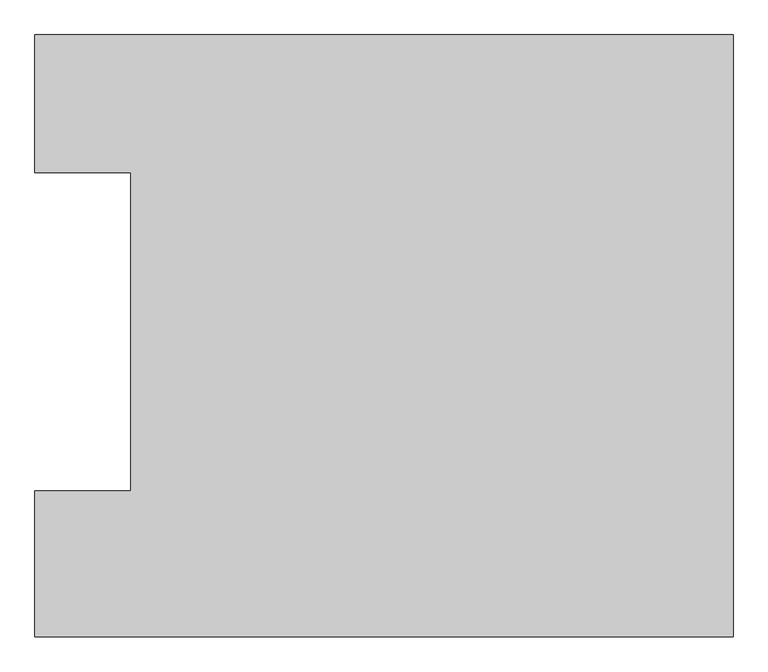
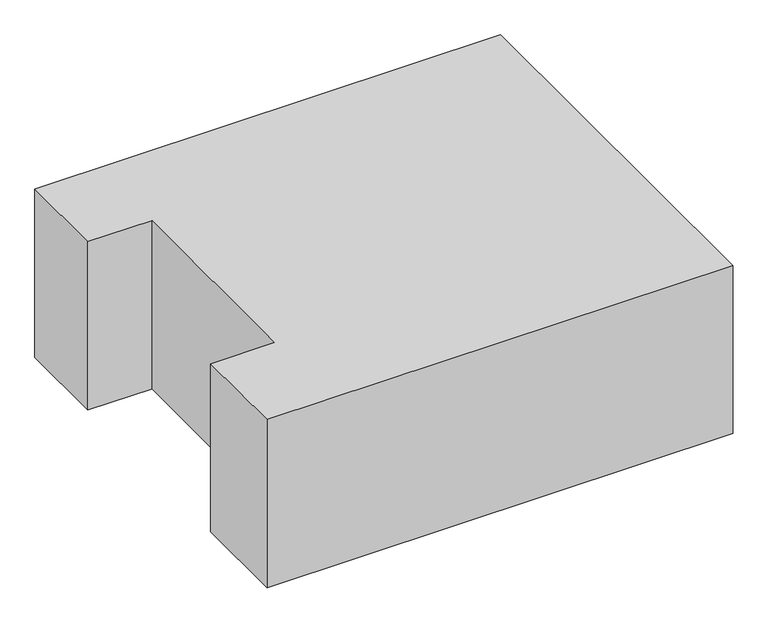
"""IFC4 building model written with IfcOpenShell, lengths in millimetres: proxy geometry, 0_3d."""

import ifcopenshell
import ifcopenshell.guid

model = None  # the IFC model being written
_history = None  # IfcOwnerHistory: only IFC2X3 demands one
_inside = {}  # id of a spatial element -> (the spatial element, [elements in it])
_under = {}  # id of a project, library or spatial element -> (it, [spatial elements below it])
_declared = {}  # id of a project -> (the project, [libraries it declares])
_typed = {}  # id of a type object -> (the type object, [elements of that type])
_made_of = {}  # id of a material, layer set ... -> (it, [elements and type objects made of it])


def new_model(schema):
    """Start an empty IFC model of exactly this schema.

    Asked for "IFC4X3", IfcOpenShell would pick the latest addendum, in which some entities
    have other attributes; the version numbers below select the first issue.
    IFC2X3 requires an IfcOwnerHistory on every rooted entity: one is made here for all.
    """
    global model, _history
    if schema == "IFC4X3":
        model = ifcopenshell.file(schema_version=(4, 3, 0, 0))
    else:
        model = ifcopenshell.file(schema=schema)
    _inside.clear()
    _under.clear()
    _declared.clear()
    _typed.clear()
    _made_of.clear()
    _history = None
    if model.schema == "IFC2X3":
        org = make("IfcOrganization", Name="unknown")
        user = make(
            "IfcPersonAndOrganization",
            ThePerson=make("IfcPerson", FamilyName="unknown"),
            TheOrganization=org,
        )
        app = make(
            "IfcApplication",
            ApplicationDeveloper=org,
            Version="unknown",
            ApplicationFullName="unknown",
            ApplicationIdentifier="unknown",
        )
        _history = make(
            "IfcOwnerHistory",
            OwningUser=user,
            OwningApplication=app,
            ChangeAction="ADDED",
            CreationDate=0,
        )
    return model


def make(cls, **values):
    """One entity of the class cls with the attributes given. An attribute that is None is left unset."""
    return model.create_entity(
        cls, **{name: value for name, value in values.items() if value is not None}
    )


def rooted(cls, **values):
    """An entity with a GlobalId (a new one), such as an element, a storey or a relation."""
    return make(cls, GlobalId=ifcopenshell.guid.new(), OwnerHistory=_history, **values)


def si_unit(unit_type, name, prefix=None):
    """IfcSIUnit, for example si_unit("LENGTHUNIT", "METRE", prefix="MILLI")."""
    return make("IfcSIUnit", UnitType=unit_type, Prefix=prefix, Name=name)


def assignment(units):
    """IfcUnitAssignment: the units of a project."""
    return None if units is None else make("IfcUnitAssignment", Units=units)


def point(xyz):
    """IfcCartesianPoint."""
    return None if xyz is None else make("IfcCartesianPoint", Coordinates=xyz)


def direction(xyz):
    """IfcDirection."""
    return None if xyz is None else make("IfcDirection", DirectionRatios=xyz)


def frame(location, z_axis=None, x_axis=None):
    """IfcAxis2Placement3D, a coordinate frame: its origin and axes. An axis left out is left unset."""
    return make(
        "IfcAxis2Placement3D",
        Location=point(location),
        Axis=direction(z_axis),
        RefDirection=direction(x_axis),
    )


def origin():
    """The frame at (0, 0, 0) with its axes left unset."""
    return frame((0.0, 0.0, 0.0))


def origin_with_axes():
    """The frame at (0, 0, 0) with the z axis (0, 0, 1) and the x axis (1, 0, 0) written out."""
    return frame((0.0, 0.0, 0.0), z_axis=(0.0, 0.0, 1.0), x_axis=(1.0, 0.0, 0.0))


def place(relative_to, where):
    """IfcLocalPlacement: puts the frame where relative to a parent placement (None: the world)."""
    return make(
        "IfcLocalPlacement", PlacementRelTo=relative_to, RelativePlacement=where
    )


def context(
    kind, dimensions, precision=None, world=None, true_north=None, identifier=None
):
    """IfcGeometricRepresentationContext, for example the 3D "Model" context."""
    return make(
        "IfcGeometricRepresentationContext",
        ContextIdentifier=identifier,
        ContextType=kind,
        CoordinateSpaceDimension=dimensions,
        Precision=precision,
        WorldCoordinateSystem=world,
        TrueNorth=true_north,
    )


def project(units=None, contexts=None):
    """IfcProject with its units and contexts."""
    return rooted(
        "IfcProject",
        Name="project",
        RepresentationContexts=contexts,
        UnitsInContext=assignment(units),
    )


def spatial(cls, under=None, at=None, **own):
    """A site, building, storey or space (cls), placed at a placement, below another one or the project."""
    s = rooted(cls, ObjectPlacement=at, **own)
    if under is not None:
        _under.setdefault(under.id(), (under, []))[1].append(s)
    return s


def polyline(points):
    """IfcPolyline through the points."""
    return make("IfcPolyline", Points=[point(p) for p in points])


def outline(outer, holes=None, kind="AREA"):
    """IfcArbitraryClosedProfileDef: a profile drawn as a closed curve; with holes, ...WithVoids."""
    if holes is None:
        return make("IfcArbitraryClosedProfileDef", ProfileType=kind, OuterCurve=outer)
    return make(
        "IfcArbitraryProfileDefWithVoids",
        ProfileType=kind,
        OuterCurve=outer,
        InnerCurves=holes,
    )


def extrude(swept, where, along, depth):
    """IfcExtrudedAreaSolid: the profile swept, set in the frame where, extruded along a direction by depth."""
    return make(
        "IfcExtrudedAreaSolid",
        SweptArea=swept,
        Position=where,
        ExtrudedDirection=direction(along),
        Depth=depth,
    )


def shape(context_of_items, identifier, shape_type, items):
    """IfcShapeRepresentation: the items that make up one representation, for example the "Body"."""
    return make(
        "IfcShapeRepresentation",
        ContextOfItems=context_of_items,
        RepresentationIdentifier=identifier,
        RepresentationType=shape_type,
        Items=items,
    )


def source(mapping_origin, context_of_items, identifier, shape_type, items):
    """IfcRepresentationMap: a shape defined once, which mapped items show again and again."""
    return make(
        "IfcRepresentationMap",
        MappingOrigin=mapping_origin,
        MappedRepresentation=shape(context_of_items, identifier, shape_type, items),
    )


def transform(
    local_origin,
    x_axis=None,
    y_axis=None,
    z_axis=None,
    scale=None,
    scale2=None,
    scale3=None,
    uniform=True,
):
    """IfcCartesianTransformationOperator3D, or its non-uniform kind. x_axis, y_axis, z_axis: its Axis1, 2, 3."""
    if uniform:
        return make(
            "IfcCartesianTransformationOperator3D",
            Axis1=direction(x_axis),
            Axis2=direction(y_axis),
            LocalOrigin=point(local_origin),
            Scale=scale,
            Axis3=direction(z_axis),
        )
    return make(
        "IfcCartesianTransformationOperator3DnonUniform",
        Axis1=direction(x_axis),
        Axis2=direction(y_axis),
        LocalOrigin=point(local_origin),
        Scale=scale,
        Axis3=direction(z_axis),
        Scale2=scale2,
        Scale3=scale3,
    )


def mapped(mapping_source, mapping_target):
    """IfcMappedItem: shows the shape of a source again, moved by a transform."""
    return make(
        "IfcMappedItem", MappingSource=mapping_source, MappingTarget=mapping_target
    )


def made_of(thing, what):
    """Note that an element or type object is made of a material, layer set ...; save() writes the relation."""
    if what is not None:
        _made_of.setdefault(what.id(), (what, []))[1].append(thing)
    return thing


def element(
    cls,
    number,
    at=None,
    inside=None,
    cuts=None,
    type_object=None,
    material=None,
    context=None,
    identifier="Body",
    shape_type=None,
    held_by="IfcProductDefinitionShape",
    body=None,
    shapes=None,
    **own,
):
    """One element of the class cls, such as IfcWall. Its Tag is "e" and its number.

    at: its placement. inside: the storey or other place that contains it. cuts: it is an
    opening in that element (IfcRelVoidsElement). A single representation is given by context,
    identifier, shape_type and body (its items); several are given by shapes. held_by: the class
    of the entity that holds the representations. save() writes the other relations.
    """
    e = rooted(cls, Tag="e%d" % number, ObjectPlacement=at, **own)
    if body is not None:
        shapes = [shape(context, identifier, shape_type, body)]
    if shapes is not None:
        e.Representation = make(held_by, Representations=shapes)
    if inside is not None:
        _inside.setdefault(inside.id(), (inside, []))[1].append(e)
    if cuts is not None:
        rooted(
            "IfcRelVoidsElement", RelatingBuildingElement=cuts, RelatedOpeningElement=e
        )
    if type_object is not None:
        _typed.setdefault(type_object.id(), (type_object, []))[1].append(e)
    return made_of(e, material)


def aggregate(whole, parts):
    """IfcRelAggregates: a whole, such as a stair, and the parts it consists of."""
    return rooted("IfcRelAggregates", RelatingObject=whole, RelatedObjects=parts)


def save(model, path):
    """Write the relations noted so far, then the file.

    IfcRelAggregates (storeys below a building ...), IfcRelContainedInSpatialStructure (elements
    in a storey), IfcRelDefinesByType, IfcRelAssociatesMaterial and IfcRelDeclares: one each for
    every whole, place, type object, material and project.
    """
    for whole, parts in _under.values():
        aggregate(whole, parts)
    for where, things in _inside.values():
        rooted(
            "IfcRelContainedInSpatialStructure",
            RelatedElements=things,
            RelatingStructure=where,
        )
    for kind, things in _typed.values():
        rooted("IfcRelDefinesByType", RelatedObjects=things, RelatingType=kind)
    for what, things in _made_of.values():
        rooted("IfcRelAssociatesMaterial", RelatedObjects=things, RelatingMaterial=what)
    for by, libraries in _declared.values():
        rooted("IfcRelDeclares", RelatingContext=by, RelatedDefinitions=libraries)
    model.write(path)


def generic_models_1e1fada3(model_context):
    return source(origin(), model_context, "Body", "SweptSolid", [
        extrude(outline(polyline([(0.0, 0.0), (0.0, 1367.8), (900.0, 1367.8), (900.0, 4357.8), (0.0, 4357.8), (0.0, 5650.0), (6550.0, 5650.0), (6550.0, 0.0), (0.0, 0.0)])), origin_with_axes(), (0.0, 0.0, 1.0), 2500.0),
    ])


if __name__ == "__main__":
    model = new_model("IFC4")
    model_context = context("Model", 3, world=origin())
    ifc_project = project(units=[si_unit("LENGTHUNIT", "METRE", prefix="MILLI")], contexts=[model_context])
    site = spatial("IfcSite", under=ifc_project)
    building = spatial("IfcBuilding", under=site)
    placement = place(None, origin())
    generic_models_shape = generic_models_1e1fada3(model_context)
    element("IfcBuildingElementProxy", 1, Name="0_3d", ObjectType="0_3d", at=placement, inside=building, context=model_context, shape_type="MappedRepresentation", body=[
        mapped(generic_models_shape, transform((0.0, 0.0, 0.0), x_axis=(1.0, 0.0, 0.0), y_axis=(0.0, 1.0, 0.0), z_axis=(0.0, 0.0, 1.0))),
    ])
    save(model, "model.ifc")

# Revit data of these elements
# Element 1 (IfcBuildingElementProxy, "0_3d")
#   Materials on its faces: "*1"
# Materials
#   "*1": class "Unassigned", colour RGB 175 175 175, transparency 0
